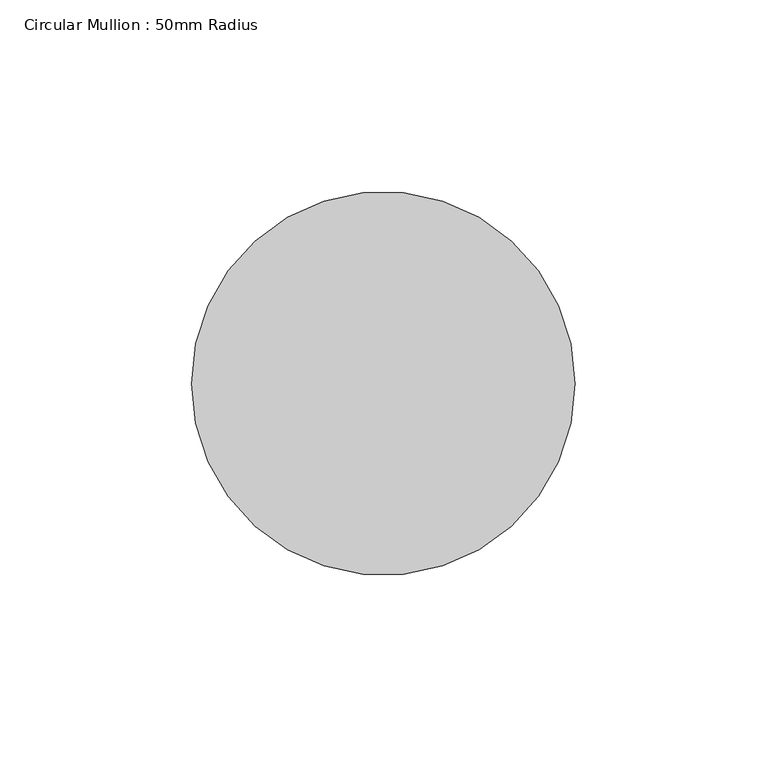
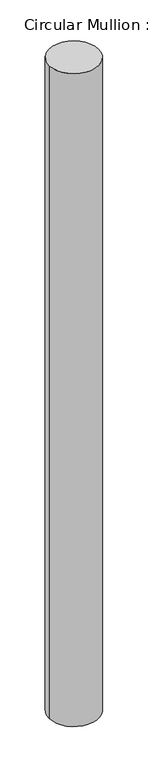
"""IFC4 building model written with IfcOpenShell, lengths in millimetres: member geometry, Circular Mullion : 50mm Radius."""

from ifc_helpers import new_model, si_unit, point, frame, origin, origin_2d, place, context, project, spatial, circle_curve, trimmed, segment, composite_curve, outline, extrude, source, transform, mapped, element, save


def circular_mullion_50mm_radius_badadaba(model_context):
    return source(origin(), model_context, "Body", "SweptSolid", [
        extrude(outline(composite_curve([segment(trimmed(circle_curve(origin_2d(), 50.0), [point((50.0, 0.0))], [point((-50.0, 0.0))], False, "CARTESIAN"), True, "CONTINUOUS"), segment(trimmed(circle_curve(origin_2d(), 50.0), [point((-50.0, 0.0))], [point((50.0, 0.0))], False, "CARTESIAN"), True, "CONTINUOUS")], self_intersect=False)), frame((0.0, 0.0, -1389.6725788), z_axis=(0.0, 0.0, 1.0), x_axis=(1.0, 0.0, 0.0)), (0.0, 0.0, 1.0), 1389.6725788),
    ])


if __name__ == "__main__":
    model = new_model("IFC4")
    model_context = context("Model", 3, world=origin())
    ifc_project = project(units=[si_unit("LENGTHUNIT", "METRE", prefix="MILLI")], contexts=[model_context])
    site = spatial("IfcSite", under=ifc_project)
    building = spatial("IfcBuilding", under=site)
    placement = place(None, origin())
    circular_mullion_50mm_radius_shape = circular_mullion_50mm_radius_badadaba(model_context)
    element("IfcMember", 1, ObjectType="Circular Mullion : 50mm Radius", at=placement, inside=building, context=model_context, shape_type="MappedRepresentation", body=[
        mapped(circular_mullion_50mm_radius_shape, transform((0.0, 0.0, 0.0), x_axis=(1.0, 0.0, 0.0), y_axis=(0.0, 1.0, 0.0), z_axis=(0.0, 0.0, 1.0))),
    ])
    save(model, "model.ifc")

# Revit data of these elements
# Type "Circular Mullion : 50mm Radius"
#   built-in parameter 1007350 = 0.164042 (stored number, unit not read)
# Element 1 (IfcMember, "Circular Mullion : 50mm Radius")
#   Materials on its faces: "Aluminium"
# Materials
#   "Aluminium": class "Metal", colour RGB 247 247 247, transparency 0, Description = "Aluminium 6061", Cost = 0
